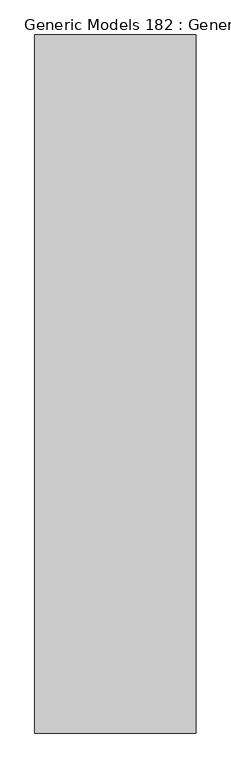
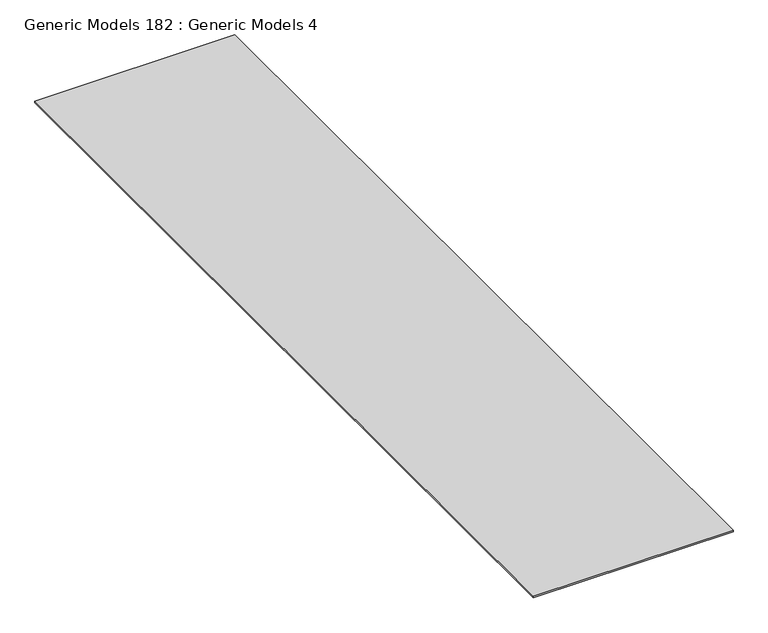
"""IFC4 building model written with IfcOpenShell, lengths in millimetres: proxy geometry, Generic Models 182 : Generic Models 4."""

from ifc_helpers import new_model, si_unit, frame, origin, place, context, project, spatial, polyline, outline, extrude, source, transform, mapped, element, save


def generic_models_182_generic_models_4_1d5b9f7e(model_context):
    return source(origin(), model_context, "Body", "SweptSolid", [
        extrude(outline(polyline([(-5328.417113, -464.1230338), (-8159.9236296, -464.1230338), (-8159.9236296, 11778.6769662), (-5328.417113, 11778.6769662), (-5328.417113, -464.1230338)])), frame((0.0, 0.0, 126767.971), z_axis=(0.0, 0.0, 1.0), x_axis=(1.0, 0.0, 0.0)), (0.0, 0.0, 1.0), 25.4),
    ])


if __name__ == "__main__":
    model = new_model("IFC4")
    model_context = context("Model", 3, world=origin())
    ifc_project = project(units=[si_unit("LENGTHUNIT", "METRE", prefix="MILLI")], contexts=[model_context])
    site = spatial("IfcSite", under=ifc_project)
    building = spatial("IfcBuilding", under=site)
    placement = place(None, origin())
    generic_models_182_generic_models_4_shape = generic_models_182_generic_models_4_1d5b9f7e(model_context)
    element("IfcBuildingElementProxy", 1, Name="Generic Models 182 : Generic Models 4", ObjectType="Generic Models 182 : Generic Models 4", at=placement, inside=building, context=model_context, shape_type="MappedRepresentation", body=[
        mapped(generic_models_182_generic_models_4_shape, transform((0.0, 0.0, 0.0), x_axis=(1.0, 0.0, 0.0), y_axis=(0.0, 1.0, 0.0), z_axis=(0.0, 0.0, 1.0))),
    ])
    save(model, "model.ifc")

# Revit data of these elements
# Element 1 (IfcBuildingElementProxy, "Generic Models 182 : Generic Models 4")
#   Materials on its faces: "_COMPOSITE DECKING"
# Materials
#   "_COMPOSITE DECKING": class "Generic", colour RGB 135 85 92, transparency 0, Cost = 0
